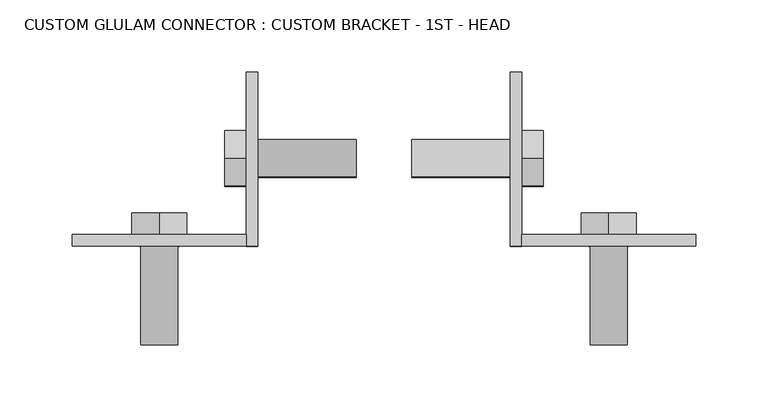
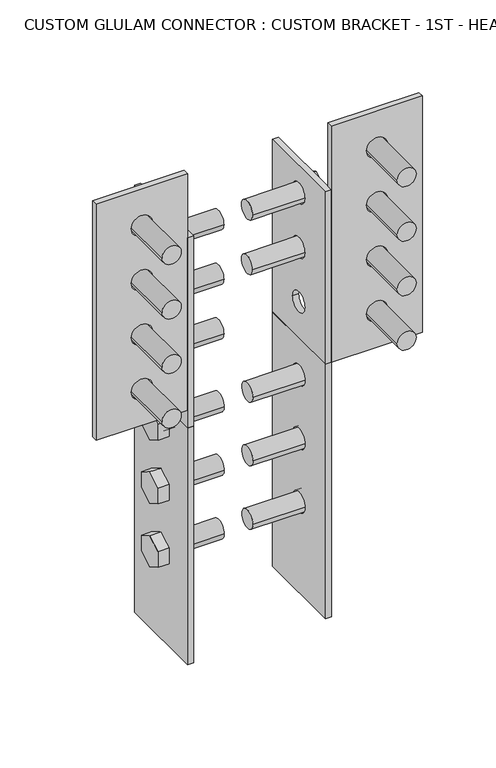
"""IFC4 building model written with IfcOpenShell, lengths in millimetres: fastener geometry, CUSTOM GLULAM CONNECTOR : CUSTOM BRACKET - 1ST - HEAD."""

from ifc_helpers import new_model, si_unit, point, frame, frame_2d, origin, place, context, project, spatial, polyline, circle_curve, trimmed, segment, composite_curve, outline, extrude, source, transform, mapped, element, save
from ifc_brep_helpers import plane_surface, revolved_surface, advanced_brep


def custom_glulam_connector_custom_bracket_1st_head_4a4bef05(model_context):
    return source(origin(), model_context, "Body", "SolidModel", [
        advanced_brep(
        [(-95.25, -60.325, 7.9375), (-87.3125, -60.325, 7.9375), (-87.3125, -60.325, 338.1375), (-95.25, -60.325, 338.1375), (-87.3125, 60.325, 7.9375), (-95.25, 60.325, 7.9375), (-95.25, 60.325, 338.1375), (-87.3125, 60.325, 338.1375), (-95.25, -13.890625, 223.8375), (-95.25, 13.890625, 223.8375), (-87.3125, 13.890625, 223.8375), (-87.3125, -13.890625, 223.8375), (-95.25, 52.3875, 7.9375), (-95.25, 13.890625, 312.7375), (-95.25, -13.890625, 312.7375), (-95.25, -13.890625, 134.9375), (-95.25, 13.890625, 134.9375), (-87.3125, -13.890625, 312.7375), (-87.3125, 13.890625, 312.7375), (-87.3125, 13.890625, 134.9375), (-87.3125, -13.890625, 134.9375)],
        [
            (0, 1),
            (1, 2),
            (2, 3),
            (3, 0),
            (4, 5),
            (5, 6),
            (6, 7),
            (7, 4),
            (8, 9, circle_curve(frame((-95.25, 0.0, 223.8375), z_axis=(-1.0, 0.0, 0.0), x_axis=(0.0, 1.0, 0.0)), 13.890625)),
            (9, 10),
            (10, 11, circle_curve(frame((-87.3125, 0.0, 223.8375), z_axis=(1.0, 0.0, 0.0), x_axis=(0.0, 1.0, 0.0)), 13.890625)),
            (11, 8),
            (5, 12),
            (12, 0),
            (3, 6),
            (8, 9, circle_curve(frame((-95.25, 0.0, 223.8375), z_axis=(1.0, 0.0, 0.0), x_axis=(0.0, 1.0, 0.0)), 13.890625)),
            (13, 14, circle_curve(frame((-95.25, 0.0, 312.7375), z_axis=(1.0, 0.0, 0.0), x_axis=(0.0, 1.0, 0.0)), 13.890625)),
            (14, 13, circle_curve(frame((-95.25, 0.0, 312.7375), z_axis=(1.0, 0.0, 0.0), x_axis=(0.0, 1.0, 0.0)), 13.890625)),
            (15, 16, circle_curve(frame((-95.25, 0.0, 134.9375), z_axis=(1.0, 0.0, 0.0), x_axis=(0.0, 1.0, 0.0)), 13.890625)),
            (16, 15, circle_curve(frame((-95.25, 0.0, 134.9375), z_axis=(1.0, 0.0, 0.0), x_axis=(0.0, 1.0, 0.0)), 13.890625)),
            (14, 17),
            (17, 18, circle_curve(frame((-87.3125, 0.0, 312.7375), z_axis=(1.0, 0.0, 0.0), x_axis=(0.0, 1.0, 0.0)), 13.890625)),
            (18, 13),
            (18, 17, circle_curve(frame((-87.3125, 0.0, 312.7375), z_axis=(1.0, 0.0, 0.0), x_axis=(0.0, 1.0, 0.0)), 13.890625)),
            (11, 10, circle_curve(frame((-87.3125, 0.0, 223.8375), z_axis=(1.0, 0.0, 0.0), x_axis=(0.0, 1.0, 0.0)), 13.890625)),
            (1, 4),
            (7, 2),
            (19, 20, circle_curve(frame((-87.3125, 0.0, 134.9375), z_axis=(-1.0, 0.0, 0.0), x_axis=(0.0, 1.0, 0.0)), 13.890625)),
            (20, 19, circle_curve(frame((-87.3125, 0.0, 134.9375), z_axis=(-1.0, 0.0, 0.0), x_axis=(0.0, 1.0, 0.0)), 13.890625)),
            (15, 20),
            (19, 16),
        ],
        [
            plane_surface(frame((-95.25, -60.325, 363.5375), z_axis=(0.0, -1.0, 0.0), x_axis=(1.0, 0.0, 0.0))),
            plane_surface(frame((-95.25, 60.325, 7.9375), z_axis=(0.0, 1.0, 0.0), x_axis=(1.0, 0.0, 0.0))),
            revolved_surface(polyline([(-95.25, 13.890625, 223.8375), (-87.3125, 13.890625, 223.8375)]), (-87.3125, 0.0, 223.8375), (-1.0, 0.0, 0.0)),
            plane_surface(frame((-95.25, -60.325, 363.5375), z_axis=(-1.0, 0.0, 0.0), x_axis=(0.0, -1.0, 0.0))),
            revolved_surface(polyline([(-95.25, 13.890625, 312.7375), (-87.3125, 13.890625, 312.7375)]), (-87.3125, 0.0, 312.7375), (-1.0, 0.0, 0.0)),
            plane_surface(frame((-87.3125, -60.325, 363.5375), z_axis=(1.0, 0.0, 0.0), x_axis=(0.0, 1.0, 0.0))),
            plane_surface(frame((-95.25, -60.325, 7.9375), z_axis=(0.0, 0.0, -1.0), x_axis=(1.0, 0.0, 0.0))),
            revolved_surface(polyline([(-95.25, 13.890625, 134.9375), (-87.3125, 13.890625, 134.9375)]), (-87.3125, 0.0, 134.9375), (-1.0, 0.0, 0.0)),
            plane_surface(frame((-95.25, -60.325, 338.1375), z_axis=(0.0, 0.0, 1.0), x_axis=(1.0, 0.0, 0.0))),
        ],
        [
            (0, [[1, 2, 3, 4]]),
            (1, [[5, 6, 7, 8]]),
            (2, [[9, 10, 11, 12]]),
            (3, [[13, 14, -4, 15, -6], [-9, 16], [17, 18], [19, 20]]),
            (4, [[-18, 21, 22, 23]]),
            (4, [[-17, -23, 24, -21]]),
            (2, [[-16, -12, 25, -10]]),
            (5, [[26, -8, 27, -2], [-24, -22], [-11, -25], [28, 29]]),
            (6, [[-14, -13, -5, -26, -1]]),
            (7, [[-19, 30, -28, 31]]),
            (7, [[-30, -20, -31, -29]]),
            (8, [[-15, -3, -27, -7]]),
        ],
    ),
        extrude(outline(polyline([(-19.05, 323.7360226), (0.0, 334.7345453), (19.05, 323.7360226), (19.05, 301.7389774), (0.0, 290.7404547), (-19.05, 301.7389774), (-19.05, 323.7360226)])), frame((-110.2320312, 0.0, 0.0), z_axis=(1.0, 0.0, 0.0), x_axis=(0.0, 1.0, 0.0)), (0.0, 0.0, 1.0), 14.9820312),
        extrude(outline(composite_curve([segment(trimmed(circle_curve(frame_2d((0.0, 312.7375)), 12.7), [point((-12.7, 312.7375))], [point((12.7, 312.7375))], False, "CARTESIAN"), True, "CONTINUOUS"), segment(trimmed(circle_curve(frame_2d((0.0, 312.7375)), 12.7), [point((12.7, 312.7375))], [point((-12.7, 312.7375))], False, "CARTESIAN"), True, "CONTINUOUS")], self_intersect=False)), frame((-95.25, 0.0, 0.0), z_axis=(1.0, 0.0, 0.0), x_axis=(0.0, 1.0, 0.0)), (0.0, 0.0, 1.0), 76.2),
        extrude(outline(polyline([(-19.05, 234.8360226), (0.0, 245.8345453), (19.05, 234.8360226), (19.05, 212.8389774), (0.0, 201.8404547), (-19.05, 212.8389774), (-19.05, 234.8360226)])), frame((-110.2320312, 0.0, 0.0), z_axis=(1.0, 0.0, 0.0), x_axis=(0.0, 1.0, 0.0)), (0.0, 0.0, 1.0), 14.9820312),
        extrude(outline(composite_curve([segment(trimmed(circle_curve(frame_2d((0.0, 223.8375)), 12.7), [point((-12.7, 223.8375))], [point((12.7, 223.8375))], False, "CARTESIAN"), True, "CONTINUOUS"), segment(trimmed(circle_curve(frame_2d((0.0, 223.8375)), 12.7), [point((12.7, 223.8375))], [point((-12.7, 223.8375))], False, "CARTESIAN"), True, "CONTINUOUS")], self_intersect=False)), frame((-95.25, 0.0, 0.0), z_axis=(1.0, 0.0, 0.0), x_axis=(0.0, 1.0, 0.0)), (0.0, 0.0, 1.0), 76.2),
        extrude(outline(polyline([(-19.05, 323.7360226), (0.0, 334.7345453), (19.05, 323.7360226), (19.05, 301.7389774), (0.0, 290.7404547), (-19.05, 301.7389774), (-19.05, 323.7360226)])), frame((-110.2320312, 0.0, 0.0), z_axis=(1.0, 0.0, 0.0), x_axis=(0.0, 1.0, 0.0)), (0.0, 0.0, 1.0), 14.9820312),
        extrude(outline(composite_curve([segment(trimmed(circle_curve(frame_2d((0.0, 312.7375)), 12.7), [point((-12.7, 312.7375))], [point((12.7, 312.7375))], False, "CARTESIAN"), True, "CONTINUOUS"), segment(trimmed(circle_curve(frame_2d((0.0, 312.7375)), 12.7), [point((12.7, 312.7375))], [point((-12.7, 312.7375))], False, "CARTESIAN"), True, "CONTINUOUS")], self_intersect=False)), frame((-95.25, 0.0, 0.0), z_axis=(1.0, 0.0, 0.0), x_axis=(0.0, 1.0, 0.0)), (0.0, 0.0, 1.0), 76.2),
        extrude(outline(polyline([(-19.05, 145.9360226), (0.0, 156.9345453), (19.05, 145.9360226), (19.05, 123.9389774), (0.0, 112.9404547), (-19.05, 123.9389774), (-19.05, 145.9360226)])), frame((-110.2320312, 0.0, 0.0), z_axis=(1.0, 0.0, 0.0), x_axis=(0.0, 1.0, 0.0)), (0.0, 0.0, 1.0), 14.9820312),
        extrude(outline(composite_curve([segment(trimmed(circle_curve(frame_2d((0.0, 134.9375)), 12.7), [point((-12.7, 134.9375))], [point((12.7, 134.9375))], False, "CARTESIAN"), True, "CONTINUOUS"), segment(trimmed(circle_curve(frame_2d((0.0, 134.9375)), 12.7), [point((12.7, 134.9375))], [point((-12.7, 134.9375))], False, "CARTESIAN"), True, "CONTINUOUS")], self_intersect=False)), frame((-95.25, 0.0, 0.0), z_axis=(1.0, 0.0, 0.0), x_axis=(0.0, 1.0, 0.0)), (0.0, 0.0, 1.0), 76.2),
        advanced_brep(
        [(95.25, -60.325, 7.9375), (95.25, -60.325, 363.5375), (87.3125, -60.325, 363.5375), (87.3125, -60.325, 7.9375), (95.25, 60.325, 363.5375), (95.25, 60.325, 7.9375), (87.3125, 60.325, 7.9375), (87.3125, 60.325, 363.5375), (95.25, -13.890625, 223.8375), (87.3125, -13.890625, 223.8375), (87.3125, 13.890625, 223.8375), (95.25, 13.890625, 223.8375), (95.25, 52.3875, 363.5375), (95.25, 52.3875, 7.9375), (95.25, 13.890625, 312.7375), (95.25, -13.890625, 312.7375), (95.25, 13.890625, 134.9375), (95.25, -13.890625, 134.9375), (87.3125, -13.890625, 312.7375), (87.3125, 13.890625, 312.7375), (87.3125, -13.890625, 134.9375), (87.3125, 13.890625, 134.9375)],
        [
            (0, 1),
            (1, 2),
            (2, 3),
            (3, 0),
            (4, 5),
            (5, 6),
            (6, 7),
            (7, 4),
            (8, 9),
            (9, 10, circle_curve(frame((87.3125, 0.0, 223.8375), z_axis=(-1.0, 0.0, 0.0), x_axis=(0.0, 1.0, 0.0)), 13.890625)),
            (10, 11),
            (11, 8, circle_curve(frame((95.25, 0.0, 223.8375), z_axis=(1.0, 0.0, 0.0), x_axis=(0.0, 1.0, 0.0)), 13.890625)),
            (4, 12),
            (12, 1),
            (0, 13),
            (13, 5),
            (14, 15, circle_curve(frame((95.25, 0.0, 312.7375), z_axis=(-1.0, 0.0, 0.0), x_axis=(0.0, 1.0, 0.0)), 13.890625)),
            (15, 14, circle_curve(frame((95.25, 0.0, 312.7375), z_axis=(-1.0, 0.0, 0.0), x_axis=(0.0, 1.0, 0.0)), 13.890625)),
            (11, 8, circle_curve(frame((95.25, 0.0, 223.8375), z_axis=(-1.0, 0.0, 0.0), x_axis=(0.0, 1.0, 0.0)), 13.890625)),
            (16, 17, circle_curve(frame((95.25, 0.0, 134.9375), z_axis=(-1.0, 0.0, 0.0), x_axis=(0.0, 1.0, 0.0)), 13.890625)),
            (17, 16, circle_curve(frame((95.25, 0.0, 134.9375), z_axis=(-1.0, 0.0, 0.0), x_axis=(0.0, 1.0, 0.0)), 13.890625)),
            (18, 15),
            (14, 19),
            (19, 18, circle_curve(frame((87.3125, 0.0, 312.7375), z_axis=(-1.0, 0.0, 0.0), x_axis=(0.0, 1.0, 0.0)), 13.890625)),
            (18, 19, circle_curve(frame((87.3125, 0.0, 312.7375), z_axis=(-1.0, 0.0, 0.0), x_axis=(0.0, 1.0, 0.0)), 13.890625)),
            (10, 9, circle_curve(frame((87.3125, 0.0, 223.8375), z_axis=(-1.0, 0.0, 0.0), x_axis=(0.0, 1.0, 0.0)), 13.890625)),
            (6, 3),
            (2, 7),
            (20, 21, circle_curve(frame((87.3125, 0.0, 134.9375), z_axis=(1.0, 0.0, 0.0), x_axis=(0.0, 1.0, 0.0)), 13.890625)),
            (21, 20, circle_curve(frame((87.3125, 0.0, 134.9375), z_axis=(1.0, 0.0, 0.0), x_axis=(0.0, 1.0, 0.0)), 13.890625)),
            (20, 17),
            (16, 21),
        ],
        [
            plane_surface(frame((95.25, -60.325, 363.5375), z_axis=(0.0, -1.0, 0.0), x_axis=(-1.0, 0.0, 0.0))),
            plane_surface(frame((95.25, 60.325, 7.9375), z_axis=(0.0, 1.0, 0.0), x_axis=(-1.0, 0.0, 0.0))),
            revolved_surface(polyline([(95.25, 13.890625, 223.8375), (87.3125, 13.890625, 223.8375)]), (87.3125, 0.0, 223.8375), (1.0, 0.0, 0.0)),
            plane_surface(frame((95.25, -60.325, 363.5375), z_axis=(1.0, 0.0, 0.0), x_axis=(0.0, -1.0, 0.0))),
            revolved_surface(polyline([(95.25, 13.890625, 312.7375), (87.3125, 13.890625, 312.7375)]), (87.3125, 0.0, 312.7375), (1.0, 0.0, 0.0)),
            plane_surface(frame((87.3125, -60.325, 363.5375), z_axis=(-1.0, 0.0, 0.0), x_axis=(0.0, 1.0, 0.0))),
            plane_surface(frame((95.25, 60.325, 363.5375), z_axis=(0.0, 0.0, 1.0), x_axis=(-1.0, 0.0, 0.0))),
            plane_surface(frame((95.25, -60.325, 7.9375), z_axis=(0.0, 0.0, -1.0), x_axis=(-1.0, 0.0, 0.0))),
            revolved_surface(polyline([(95.25, 13.890625, 134.9375), (87.3125, 13.890625, 134.9375)]), (87.3125, 0.0, 134.9375), (1.0, 0.0, 0.0)),
        ],
        [
            (0, [[1, 2, 3, 4]]),
            (1, [[5, 6, 7, 8]]),
            (2, [[9, 10, 11, 12]]),
            (3, [[13, 14, -1, 15, 16, -5], [17, 18], [19, -12], [20, 21]]),
            (4, [[22, -17, 23, 24]]),
            (4, [[-22, 25, -23, -18]]),
            (2, [[-9, -19, -11, 26]]),
            (5, [[-7, 27, -3, 28], [-24, -25], [-26, -10], [29, 30]]),
            (6, [[-14, -13, -8, -28, -2]]),
            (7, [[-16, -15, -4, -27, -6]]),
            (8, [[31, -20, 32, -29]]),
            (8, [[-31, -30, -32, -21]]),
        ],
    ),
        extrude(outline(polyline([(-19.05, 323.7360226), (0.0, 334.7345453), (19.05, 323.7360226), (19.05, 301.7389774), (0.0, 290.7404547), (-19.05, 301.7389774), (-19.05, 323.7360226)])), frame((95.25, 0.0, 0.0), z_axis=(1.0, 0.0, 0.0), x_axis=(0.0, 1.0, 0.0)), (0.0, 0.0, 1.0), 14.9820312),
        extrude(outline(composite_curve([segment(trimmed(circle_curve(frame_2d((0.0, 312.7375)), 12.7), [point((-12.7, 312.7375))], [point((12.7, 312.7375))], False, "CARTESIAN"), True, "CONTINUOUS"), segment(trimmed(circle_curve(frame_2d((0.0, 312.7375)), 12.7), [point((12.7, 312.7375))], [point((-12.7, 312.7375))], False, "CARTESIAN"), True, "CONTINUOUS")], self_intersect=False)), frame((19.05, 0.0, 0.0), z_axis=(1.0, 0.0, 0.0), x_axis=(0.0, 1.0, 0.0)), (0.0, 0.0, 1.0), 76.2),
        extrude(outline(polyline([(-19.05, 234.8360226), (0.0, 245.8345453), (19.05, 234.8360226), (19.05, 212.8389774), (0.0, 201.8404547), (-19.05, 212.8389774), (-19.05, 234.8360226)])), frame((95.25, 0.0, 0.0), z_axis=(1.0, 0.0, 0.0), x_axis=(0.0, 1.0, 0.0)), (0.0, 0.0, 1.0), 14.9820312),
        extrude(outline(composite_curve([segment(trimmed(circle_curve(frame_2d((0.0, 223.8375)), 12.7), [point((-12.7, 223.8375))], [point((12.7, 223.8375))], False, "CARTESIAN"), True, "CONTINUOUS"), segment(trimmed(circle_curve(frame_2d((0.0, 223.8375)), 12.7), [point((12.7, 223.8375))], [point((-12.7, 223.8375))], False, "CARTESIAN"), True, "CONTINUOUS")], self_intersect=False)), frame((19.05, 0.0, 0.0), z_axis=(1.0, 0.0, 0.0), x_axis=(0.0, 1.0, 0.0)), (0.0, 0.0, 1.0), 76.2),
        extrude(outline(polyline([(-19.05, 323.7360226), (0.0, 334.7345453), (19.05, 323.7360226), (19.05, 301.7389774), (0.0, 290.7404547), (-19.05, 301.7389774), (-19.05, 323.7360226)])), frame((95.25, 0.0, 0.0), z_axis=(1.0, 0.0, 0.0), x_axis=(0.0, 1.0, 0.0)), (0.0, 0.0, 1.0), 14.9820312),
        extrude(outline(composite_curve([segment(trimmed(circle_curve(frame_2d((0.0, 312.7375)), 12.7), [point((-12.7, 312.7375))], [point((12.7, 312.7375))], False, "CARTESIAN"), True, "CONTINUOUS"), segment(trimmed(circle_curve(frame_2d((0.0, 312.7375)), 12.7), [point((12.7, 312.7375))], [point((-12.7, 312.7375))], False, "CARTESIAN"), True, "CONTINUOUS")], self_intersect=False)), frame((19.05, 0.0, 0.0), z_axis=(1.0, 0.0, 0.0), x_axis=(0.0, 1.0, 0.0)), (0.0, 0.0, 1.0), 76.2),
        extrude(outline(polyline([(-19.05, 145.9360226), (0.0, 156.9345453), (19.05, 145.9360226), (19.05, 123.9389774), (0.0, 112.9404547), (-19.05, 123.9389774), (-19.05, 145.9360226)])), frame((95.25, 0.0, 0.0), z_axis=(1.0, 0.0, 0.0), x_axis=(0.0, 1.0, 0.0)), (0.0, 0.0, 1.0), 14.9820312),
        extrude(outline(composite_curve([segment(trimmed(circle_curve(frame_2d((0.0, 134.9375)), 12.7), [point((-12.7, 134.9375))], [point((12.7, 134.9375))], False, "CARTESIAN"), True, "CONTINUOUS"), segment(trimmed(circle_curve(frame_2d((0.0, 134.9375)), 12.7), [point((12.7, 134.9375))], [point((-12.7, 134.9375))], False, "CARTESIAN"), True, "CONTINUOUS")], self_intersect=False)), frame((19.05, 0.0, 0.0), z_axis=(1.0, 0.0, 0.0), x_axis=(0.0, 1.0, 0.0)), (0.0, 0.0, 1.0), 76.2),
        advanced_brep(
        [(-215.9, -52.3875, 693.7375), (-215.9, -52.3875, 363.5375), (-215.9, -60.325, 363.5375), (-215.9, -60.325, 693.7375), (-141.684375, -60.325, 642.9375), (-141.684375, -52.3875, 642.9375), (-169.465625, -52.3875, 642.9375), (-169.465625, -60.325, 642.9375), (-95.25, -52.3875, 693.7375), (-95.25, -52.3875, 363.5375), (-169.465625, -52.3875, 566.7375), (-141.684375, -52.3875, 566.7375), (-169.465625, -52.3875, 490.5375), (-141.684375, -52.3875, 490.5375), (-169.465625, -52.3875, 414.3375), (-141.684375, -52.3875, 414.3375), (-95.25, -60.325, 693.7375), (-95.25, -60.325, 604.8375), (-95.25, -60.325, 363.5375), (-141.684375, -60.325, 566.7375), (-169.465625, -60.325, 566.7375), (-141.684375, -60.325, 490.5375), (-169.465625, -60.325, 490.5375), (-141.684375, -60.325, 414.3375), (-169.465625, -60.325, 414.3375)],
        [
            (0, 1),
            (1, 2),
            (2, 3),
            (3, 0),
            (4, 5),
            (5, 6, circle_curve(frame((-155.575, -52.3875, 642.9375), z_axis=(0.0, 1.0, 0.0), x_axis=(-1.0, 0.0, 0.0)), 13.890625)),
            (6, 7),
            (7, 4, circle_curve(frame((-155.575, -60.325, 642.9375), z_axis=(0.0, -1.0, 0.0), x_axis=(-1.0, 0.0, 0.0)), 13.890625)),
            (4, 7, circle_curve(frame((-155.575, -60.325, 642.9375), z_axis=(0.0, -1.0, 0.0), x_axis=(-1.0, 0.0, 0.0)), 13.890625)),
            (6, 5, circle_curve(frame((-155.575, -52.3875, 642.9375), z_axis=(0.0, 1.0, 0.0), x_axis=(-1.0, 0.0, 0.0)), 13.890625)),
            (0, 8),
            (8, 9),
            (9, 1),
            (10, 11, circle_curve(frame((-155.575, -52.3875, 566.7375), z_axis=(0.0, -1.0, 0.0), x_axis=(-1.0, 0.0, 0.0)), 13.890625)),
            (11, 10, circle_curve(frame((-155.575, -52.3875, 566.7375), z_axis=(0.0, -1.0, 0.0), x_axis=(-1.0, 0.0, 0.0)), 13.890625)),
            (12, 13, circle_curve(frame((-155.575, -52.3875, 490.5375), z_axis=(0.0, -1.0, 0.0), x_axis=(-1.0, 0.0, 0.0)), 13.890625)),
            (13, 12, circle_curve(frame((-155.575, -52.3875, 490.5375), z_axis=(0.0, -1.0, 0.0), x_axis=(-1.0, 0.0, 0.0)), 13.890625)),
            (14, 15, circle_curve(frame((-155.575, -52.3875, 414.3375), z_axis=(0.0, -1.0, 0.0), x_axis=(-1.0, 0.0, 0.0)), 13.890625)),
            (15, 14, circle_curve(frame((-155.575, -52.3875, 414.3375), z_axis=(0.0, -1.0, 0.0), x_axis=(-1.0, 0.0, 0.0)), 13.890625)),
            (8, 16),
            (16, 17),
            (17, 18),
            (18, 9),
            (18, 2),
            (16, 3),
            (19, 20, circle_curve(frame((-155.575, -60.325, 566.7375), z_axis=(0.0, 1.0, 0.0), x_axis=(-1.0, 0.0, 0.0)), 13.890625)),
            (20, 19, circle_curve(frame((-155.575, -60.325, 566.7375), z_axis=(0.0, 1.0, 0.0), x_axis=(-1.0, 0.0, 0.0)), 13.890625)),
            (21, 22, circle_curve(frame((-155.575, -60.325, 490.5375), z_axis=(0.0, 1.0, 0.0), x_axis=(-1.0, 0.0, 0.0)), 13.890625)),
            (22, 21, circle_curve(frame((-155.575, -60.325, 490.5375), z_axis=(0.0, 1.0, 0.0), x_axis=(-1.0, 0.0, 0.0)), 13.890625)),
            (23, 24, circle_curve(frame((-155.575, -60.325, 414.3375), z_axis=(0.0, 1.0, 0.0), x_axis=(-1.0, 0.0, 0.0)), 13.890625)),
            (24, 23, circle_curve(frame((-155.575, -60.325, 414.3375), z_axis=(0.0, 1.0, 0.0), x_axis=(-1.0, 0.0, 0.0)), 13.890625)),
            (19, 11),
            (10, 20),
            (13, 21),
            (22, 12),
            (23, 15),
            (14, 24),
        ],
        [
            plane_surface(frame((-215.9, -52.3875, 363.5375), z_axis=(-1.0, 0.0, 0.0), x_axis=(0.0, -1.0, 0.0))),
            revolved_surface(polyline([(-169.465625, -52.3875, 642.9375), (-169.465625, -60.325, 642.9375)]), (-155.575, -60.325, 642.9375), (0.0, 1.0, 0.0)),
            plane_surface(frame((-95.25, -52.3875, 693.7375), z_axis=(0.0, 1.0, 0.0), x_axis=(1.0, 0.0, 0.0))),
            plane_surface(frame((-95.25, -52.3875, 693.7375), z_axis=(1.0, 0.0, 0.0), x_axis=(0.0, -1.0, 0.0))),
            plane_surface(frame((-95.25, -52.3875, 363.5375), z_axis=(0.0, 0.0, -1.0), x_axis=(0.0, -1.0, 0.0))),
            plane_surface(frame((-95.25, -60.325, 693.7375), z_axis=(0.0, -1.0, 0.0), x_axis=(-1.0, 0.0, 0.0))),
            plane_surface(frame((-215.9, -52.3875, 693.7375), z_axis=(0.0, 0.0, 1.0), x_axis=(0.0, -1.0, 0.0))),
            revolved_surface(polyline([(-169.465625, -52.3875, 566.7375), (-169.465625, -60.325, 566.7375)]), (-155.575, -60.325, 566.7375), (0.0, 1.0, 0.0)),
            revolved_surface(polyline([(-169.465625, -52.3875, 490.5375), (-169.465625, -60.325, 490.5375)]), (-155.575, -60.325, 490.5375), (0.0, 1.0, 0.0)),
            revolved_surface(polyline([(-169.465625, -52.3875, 414.3375), (-169.465625, -60.325, 414.3375)]), (-155.575, -60.325, 414.3375), (0.0, 1.0, 0.0)),
        ],
        [
            (0, [[1, 2, 3, 4]]),
            (1, [[5, 6, 7, 8]]),
            (1, [[-5, 9, -7, 10]]),
            (2, [[11, 12, 13, -1], [14, 15], [-6, -10], [16, 17], [18, 19]]),
            (3, [[-12, 20, 21, 22, 23]]),
            (4, [[-13, -23, 24, -2]]),
            (5, [[-3, -24, -22, -21, 25], [-8, -9], [26, 27], [28, 29], [30, 31]]),
            (6, [[-11, -4, -25, -20]]),
            (7, [[32, -14, 33, -26]]),
            (7, [[-32, -27, -33, -15]]),
            (8, [[34, -29, 35, -17]]),
            (8, [[-34, -16, -35, -28]]),
            (9, [[36, -18, 37, -30]]),
            (9, [[-36, -31, -37, -19]]),
        ],
    ),
        extrude(outline(polyline([(653.9360226, -136.525), (664.9345453, -155.575), (653.9360226, -174.625), (631.9389774, -174.625), (620.9404547, -155.575), (631.9389774, -136.525), (653.9360226, -136.525)])), frame((0.0, -52.3875, 0.0), z_axis=(0.0, 1.0, 0.0), x_axis=(0.0, 0.0, 1.0)), (0.0, 0.0, 1.0), 14.9820312),
        extrude(outline(composite_curve([segment(trimmed(circle_curve(frame_2d((642.9375, -155.575)), 12.7), [point((642.9375, -142.875))], [point((642.9375, -168.275))], False, "CARTESIAN"), True, "CONTINUOUS"), segment(trimmed(circle_curve(frame_2d((642.9375, -155.575)), 12.7), [point((642.9375, -168.275))], [point((642.9375, -142.875))], False, "CARTESIAN"), True, "CONTINUOUS")], self_intersect=False)), frame((0.0, -128.5875, 0.0), z_axis=(0.0, 1.0, 0.0), x_axis=(0.0, 0.0, 1.0)), (0.0, 0.0, 1.0), 76.2),
        extrude(outline(polyline([(577.7360226, -136.525), (588.7345453, -155.575), (577.7360226, -174.625), (555.7389774, -174.625), (544.7404547, -155.575), (555.7389774, -136.525), (577.7360226, -136.525)])), frame((0.0, -52.3875, 0.0), z_axis=(0.0, 1.0, 0.0), x_axis=(0.0, 0.0, 1.0)), (0.0, 0.0, 1.0), 14.9820312),
        extrude(outline(composite_curve([segment(trimmed(circle_curve(frame_2d((566.7375, -155.575)), 12.7), [point((566.7375, -142.875))], [point((566.7375, -168.275))], False, "CARTESIAN"), True, "CONTINUOUS"), segment(trimmed(circle_curve(frame_2d((566.7375, -155.575)), 12.7), [point((566.7375, -168.275))], [point((566.7375, -142.875))], False, "CARTESIAN"), True, "CONTINUOUS")], self_intersect=False)), frame((0.0, -128.5875, 0.0), z_axis=(0.0, 1.0, 0.0), x_axis=(0.0, 0.0, 1.0)), (0.0, 0.0, 1.0), 76.2),
        extrude(outline(polyline([(653.9360226, -136.525), (664.9345453, -155.575), (653.9360226, -174.625), (631.9389774, -174.625), (620.9404547, -155.575), (631.9389774, -136.525), (653.9360226, -136.525)])), frame((0.0, -52.3875, 0.0), z_axis=(0.0, 1.0, 0.0), x_axis=(0.0, 0.0, 1.0)), (0.0, 0.0, 1.0), 14.9820312),
        extrude(outline(composite_curve([segment(trimmed(circle_curve(frame_2d((642.9375, -155.575)), 12.7), [point((642.9375, -142.875))], [point((642.9375, -168.275))], False, "CARTESIAN"), True, "CONTINUOUS"), segment(trimmed(circle_curve(frame_2d((642.9375, -155.575)), 12.7), [point((642.9375, -168.275))], [point((642.9375, -142.875))], False, "CARTESIAN"), True, "CONTINUOUS")], self_intersect=False)), frame((0.0, -128.5875, 0.0), z_axis=(0.0, 1.0, 0.0), x_axis=(0.0, 0.0, 1.0)), (0.0, 0.0, 1.0), 76.2),
        extrude(outline(polyline([(501.5360226, -136.525), (512.5345453, -155.575), (501.5360226, -174.625), (479.5389774, -174.625), (468.5404547, -155.575), (479.5389774, -136.525), (501.5360226, -136.525)])), frame((0.0, -52.3875, 0.0), z_axis=(0.0, 1.0, 0.0), x_axis=(0.0, 0.0, 1.0)), (0.0, 0.0, 1.0), 14.9820312),
        extrude(outline(composite_curve([segment(trimmed(circle_curve(frame_2d((490.5375, -155.575)), 12.7), [point((490.5375, -142.875))], [point((490.5375, -168.275))], False, "CARTESIAN"), True, "CONTINUOUS"), segment(trimmed(circle_curve(frame_2d((490.5375, -155.575)), 12.7), [point((490.5375, -168.275))], [point((490.5375, -142.875))], False, "CARTESIAN"), True, "CONTINUOUS")], self_intersect=False)), frame((0.0, -128.5875, 0.0), z_axis=(0.0, 1.0, 0.0), x_axis=(0.0, 0.0, 1.0)), (0.0, 0.0, 1.0), 76.2),
        extrude(outline(polyline([(425.3360226, -136.525), (436.3345453, -155.575), (425.3360226, -174.625), (403.3389774, -174.625), (392.3404547, -155.575), (403.3389774, -136.525), (425.3360226, -136.525)])), frame((0.0, -52.3875, 0.0), z_axis=(0.0, 1.0, 0.0), x_axis=(0.0, 0.0, 1.0)), (0.0, 0.0, 1.0), 14.9820312),
        extrude(outline(composite_curve([segment(trimmed(circle_curve(frame_2d((414.3375, -155.575)), 12.7), [point((414.3375, -142.875))], [point((414.3375, -168.275))], False, "CARTESIAN"), True, "CONTINUOUS"), segment(trimmed(circle_curve(frame_2d((414.3375, -155.575)), 12.7), [point((414.3375, -168.275))], [point((414.3375, -142.875))], False, "CARTESIAN"), True, "CONTINUOUS")], self_intersect=False)), frame((0.0, -128.5875, 0.0), z_axis=(0.0, 1.0, 0.0), x_axis=(0.0, 0.0, 1.0)), (0.0, 0.0, 1.0), 76.2),
        advanced_brep(
        [(-95.25, -60.325, 338.1375), (-87.3125, -60.325, 338.1375), (-87.3125, -60.325, 604.8375), (-95.25, -60.325, 604.8375), (-95.25, -60.325, 363.5375), (-95.25, 60.325, 604.8375), (-87.3125, 60.325, 604.8375), (-87.3125, 60.325, 338.1375), (-95.25, 60.325, 338.1375), (-95.25, -13.096875, 490.5375), (-95.25, 14.684375, 490.5375), (-87.3125, 14.684375, 490.5375), (-87.3125, -13.096875, 490.5375), (-95.25, 14.684375, 566.7375), (-95.25, -13.096875, 566.7375), (-95.25, 14.684375, 414.3375), (-95.25, -13.096875, 414.3375), (-87.3125, -13.096875, 566.7375), (-87.3125, 14.684375, 566.7375), (-87.3125, -13.096875, 414.3375), (-87.3125, 14.684375, 414.3375)],
        [
            (0, 1),
            (1, 2),
            (2, 3),
            (3, 4),
            (4, 0),
            (5, 6),
            (6, 7),
            (7, 8),
            (8, 5),
            (9, 10, circle_curve(frame((-95.25, 0.79375, 490.5375), z_axis=(-1.0, 0.0, 0.0), x_axis=(0.0, 1.0, 0.0)), 13.890625)),
            (10, 11),
            (11, 12, circle_curve(frame((-87.3125, 0.79375, 490.5375), z_axis=(1.0, 0.0, 0.0), x_axis=(0.0, 1.0, 0.0)), 13.890625)),
            (12, 9),
            (8, 0),
            (3, 5),
            (9, 10, circle_curve(frame((-95.25, 0.79375, 490.5375), z_axis=(1.0, 0.0, 0.0), x_axis=(0.0, 1.0, 0.0)), 13.890625)),
            (13, 14, circle_curve(frame((-95.25, 0.79375, 566.7375), z_axis=(1.0, 0.0, 0.0), x_axis=(0.0, 1.0, 0.0)), 13.890625)),
            (14, 13, circle_curve(frame((-95.25, 0.79375, 566.7375), z_axis=(1.0, 0.0, 0.0), x_axis=(0.0, 1.0, 0.0)), 13.890625)),
            (15, 16, circle_curve(frame((-95.25, 0.79375, 414.3375), z_axis=(1.0, 0.0, 0.0), x_axis=(0.0, 1.0, 0.0)), 13.890625)),
            (16, 15, circle_curve(frame((-95.25, 0.79375, 414.3375), z_axis=(1.0, 0.0, 0.0), x_axis=(0.0, 1.0, 0.0)), 13.890625)),
            (17, 18, circle_curve(frame((-87.3125, 0.79375, 566.7375), z_axis=(1.0, 0.0, 0.0), x_axis=(0.0, 1.0, 0.0)), 13.890625)),
            (18, 13),
            (14, 17),
            (18, 17, circle_curve(frame((-87.3125, 0.79375, 566.7375), z_axis=(1.0, 0.0, 0.0), x_axis=(0.0, 1.0, 0.0)), 13.890625)),
            (12, 11, circle_curve(frame((-87.3125, 0.79375, 490.5375), z_axis=(1.0, 0.0, 0.0), x_axis=(0.0, 1.0, 0.0)), 13.890625)),
            (6, 2),
            (1, 7),
            (19, 20, circle_curve(frame((-87.3125, 0.79375, 414.3375), z_axis=(-1.0, 0.0, 0.0), x_axis=(0.0, 1.0, 0.0)), 13.890625)),
            (20, 19, circle_curve(frame((-87.3125, 0.79375, 414.3375), z_axis=(-1.0, 0.0, 0.0), x_axis=(0.0, 1.0, 0.0)), 13.890625)),
            (20, 15),
            (16, 19),
        ],
        [
            plane_surface(frame((-95.25, -60.325, 604.8375), z_axis=(0.0, -1.0, 0.0), x_axis=(1.0, 0.0, 0.0))),
            plane_surface(frame((-95.25, 60.325, 338.1375), z_axis=(0.0, 1.0, 0.0), x_axis=(1.0, 0.0, 0.0))),
            revolved_surface(polyline([(-95.25, 14.684375, 490.5375), (-87.3125, 14.684375, 490.5375)]), (-87.3125, 0.79375, 490.5375), (-1.0, 0.0, 0.0)),
            plane_surface(frame((-95.25, -60.325, 604.8375), z_axis=(-1.0, 0.0, 0.0), x_axis=(0.0, -1.0, 0.0))),
            revolved_surface(polyline([(-95.25, 14.684375, 566.7375), (-87.3125, 14.684375, 566.7375)]), (-87.3125, 0.79375, 566.7375), (-1.0, 0.0, 0.0)),
            plane_surface(frame((-87.3125, -60.325, 604.8375), z_axis=(1.0, 0.0, 0.0), x_axis=(0.0, 1.0, 0.0))),
            plane_surface(frame((-95.25, 60.325, 604.8375), z_axis=(0.0, 0.0, 1.0), x_axis=(1.0, 0.0, 0.0))),
            plane_surface(frame((-95.25, -60.325, 338.1375), z_axis=(0.0, 0.0, -1.0), x_axis=(1.0, 0.0, 0.0))),
            revolved_surface(polyline([(-95.25, 14.684375, 414.3375), (-87.3125, 14.684375, 414.3375)]), (-87.3125, 0.79375, 414.3375), (-1.0, 0.0, 0.0)),
        ],
        [
            (0, [[1, 2, 3, 4, 5]]),
            (1, [[6, 7, 8, 9]]),
            (2, [[10, 11, 12, 13]]),
            (3, [[-9, 14, -5, -4, 15], [-10, 16], [17, 18], [19, 20]]),
            (4, [[21, 22, -18, 23]]),
            (4, [[-17, -22, 24, -23]]),
            (2, [[25, -11, -16, -13]]),
            (5, [[26, -2, 27, -7], [-24, -21], [-12, -25], [28, 29]]),
            (6, [[-3, -26, -6, -15]]),
            (7, [[-8, -27, -1, -14]]),
            (8, [[-29, 30, -20, 31]]),
            (8, [[-19, -30, -28, -31]]),
        ],
    ),
        extrude(outline(polyline([(-18.25625, 577.7360226), (0.79375, 588.7345453), (19.84375, 577.7360226), (19.84375, 555.7389774), (0.79375, 544.7404547), (-18.25625, 555.7389774), (-18.25625, 577.7360226)])), frame((-110.2320312, 0.0, 0.0), z_axis=(1.0, 0.0, 0.0), x_axis=(0.0, 1.0, 0.0)), (0.0, 0.0, 1.0), 14.9820312),
        extrude(outline(composite_curve([segment(trimmed(circle_curve(frame_2d((0.79375, 566.7375)), 12.7), [point((-11.90625, 566.7375))], [point((13.49375, 566.7375))], False, "CARTESIAN"), True, "CONTINUOUS"), segment(trimmed(circle_curve(frame_2d((0.79375, 566.7375)), 12.7), [point((13.49375, 566.7375))], [point((-11.90625, 566.7375))], False, "CARTESIAN"), True, "CONTINUOUS")], self_intersect=False)), frame((-95.25, 0.0, 0.0), z_axis=(1.0, 0.0, 0.0), x_axis=(0.0, 1.0, 0.0)), (0.0, 0.0, 1.0), 76.2),
        extrude(outline(polyline([(-18.25625, 501.5360226), (0.79375, 512.5345453), (19.84375, 501.5360226), (19.84375, 479.5389774), (0.79375, 468.5404547), (-18.25625, 479.5389774), (-18.25625, 501.5360226)])), frame((-110.2320312, 0.0, 0.0), z_axis=(1.0, 0.0, 0.0), x_axis=(0.0, 1.0, 0.0)), (0.0, 0.0, 1.0), 14.9820312),
        extrude(outline(composite_curve([segment(trimmed(circle_curve(frame_2d((0.79375, 490.5375)), 12.7), [point((-11.90625, 490.5375))], [point((13.49375, 490.5375))], False, "CARTESIAN"), True, "CONTINUOUS"), segment(trimmed(circle_curve(frame_2d((0.79375, 490.5375)), 12.7), [point((13.49375, 490.5375))], [point((-11.90625, 490.5375))], False, "CARTESIAN"), True, "CONTINUOUS")], self_intersect=False)), frame((-95.25, 0.0, 0.0), z_axis=(1.0, 0.0, 0.0), x_axis=(0.0, 1.0, 0.0)), (0.0, 0.0, 1.0), 76.2),
        extrude(outline(polyline([(-18.25625, 577.7360226), (0.79375, 588.7345453), (19.84375, 577.7360226), (19.84375, 555.7389774), (0.79375, 544.7404547), (-18.25625, 555.7389774), (-18.25625, 577.7360226)])), frame((-110.2320312, 0.0, 0.0), z_axis=(1.0, 0.0, 0.0), x_axis=(0.0, 1.0, 0.0)), (0.0, 0.0, 1.0), 14.9820312),
        extrude(outline(composite_curve([segment(trimmed(circle_curve(frame_2d((0.79375, 566.7375)), 12.7), [point((-11.90625, 566.7375))], [point((13.49375, 566.7375))], False, "CARTESIAN"), True, "CONTINUOUS"), segment(trimmed(circle_curve(frame_2d((0.79375, 566.7375)), 12.7), [point((13.49375, 566.7375))], [point((-11.90625, 566.7375))], False, "CARTESIAN"), True, "CONTINUOUS")], self_intersect=False)), frame((-95.25, 0.0, 0.0), z_axis=(1.0, 0.0, 0.0), x_axis=(0.0, 1.0, 0.0)), (0.0, 0.0, 1.0), 76.2),
        extrude(outline(polyline([(-18.25625, 425.3360226), (0.79375, 436.3345453), (19.84375, 425.3360226), (19.84375, 403.3389774), (0.79375, 392.3404547), (-18.25625, 403.3389774), (-18.25625, 425.3360226)])), frame((-110.2320312, 0.0, 0.0), z_axis=(1.0, 0.0, 0.0), x_axis=(0.0, 1.0, 0.0)), (0.0, 0.0, 1.0), 14.9820312),
        extrude(outline(composite_curve([segment(trimmed(circle_curve(frame_2d((0.79375, 414.3375)), 12.7), [point((-11.90625, 414.3375))], [point((13.49375, 414.3375))], False, "CARTESIAN"), True, "CONTINUOUS"), segment(trimmed(circle_curve(frame_2d((0.79375, 414.3375)), 12.7), [point((13.49375, 414.3375))], [point((-11.90625, 414.3375))], False, "CARTESIAN"), True, "CONTINUOUS")], self_intersect=False)), frame((-95.25, 0.0, 0.0), z_axis=(1.0, 0.0, 0.0), x_axis=(0.0, 1.0, 0.0)), (0.0, 0.0, 1.0), 76.2),
        advanced_brep(
        [(215.9, -52.3875, 693.7375), (215.9, -60.325, 693.7375), (215.9, -60.325, 363.5375), (215.9, -52.3875, 363.5375), (141.684375, -60.325, 642.9375), (169.465625, -60.325, 642.9375), (169.465625, -52.3875, 642.9375), (141.684375, -52.3875, 642.9375), (95.25, -52.3875, 363.5375), (95.25, -52.3875, 693.7375), (169.465625, -52.3875, 566.7375), (141.684375, -52.3875, 566.7375), (169.465625, -52.3875, 490.5375), (141.684375, -52.3875, 490.5375), (169.465625, -52.3875, 414.3375), (141.684375, -52.3875, 414.3375), (95.25, -60.325, 363.5375), (95.25, -60.325, 604.8375), (95.25, -60.325, 693.7375), (141.684375, -60.325, 566.7375), (169.465625, -60.325, 566.7375), (141.684375, -60.325, 490.5375), (169.465625, -60.325, 490.5375), (141.684375, -60.325, 414.3375), (169.465625, -60.325, 414.3375)],
        [
            (0, 1),
            (1, 2),
            (2, 3),
            (3, 0),
            (4, 5, circle_curve(frame((155.575, -60.325, 642.9375), z_axis=(0.0, -1.0, 0.0), x_axis=(1.0, 0.0, 0.0)), 13.890625)),
            (5, 6),
            (6, 7, circle_curve(frame((155.575, -52.3875, 642.9375), z_axis=(0.0, 1.0, 0.0), x_axis=(1.0, 0.0, 0.0)), 13.890625)),
            (7, 4),
            (7, 6, circle_curve(frame((155.575, -52.3875, 642.9375), z_axis=(0.0, 1.0, 0.0), x_axis=(1.0, 0.0, 0.0)), 13.890625)),
            (5, 4, circle_curve(frame((155.575, -60.325, 642.9375), z_axis=(0.0, -1.0, 0.0), x_axis=(1.0, 0.0, 0.0)), 13.890625)),
            (3, 8),
            (8, 9),
            (9, 0),
            (10, 11, circle_curve(frame((155.575, -52.3875, 566.7375), z_axis=(0.0, -1.0, 0.0), x_axis=(1.0, 0.0, 0.0)), 13.890625)),
            (11, 10, circle_curve(frame((155.575, -52.3875, 566.7375), z_axis=(0.0, -1.0, 0.0), x_axis=(1.0, 0.0, 0.0)), 13.890625)),
            (12, 13, circle_curve(frame((155.575, -52.3875, 490.5375), z_axis=(0.0, -1.0, 0.0), x_axis=(1.0, 0.0, 0.0)), 13.890625)),
            (13, 12, circle_curve(frame((155.575, -52.3875, 490.5375), z_axis=(0.0, -1.0, 0.0), x_axis=(1.0, 0.0, 0.0)), 13.890625)),
            (14, 15, circle_curve(frame((155.575, -52.3875, 414.3375), z_axis=(0.0, -1.0, 0.0), x_axis=(1.0, 0.0, 0.0)), 13.890625)),
            (15, 14, circle_curve(frame((155.575, -52.3875, 414.3375), z_axis=(0.0, -1.0, 0.0), x_axis=(1.0, 0.0, 0.0)), 13.890625)),
            (8, 16),
            (16, 17),
            (17, 18),
            (18, 9),
            (2, 16),
            (1, 18),
            (19, 20, circle_curve(frame((155.575, -60.325, 566.7375), z_axis=(0.0, 1.0, 0.0), x_axis=(1.0, 0.0, 0.0)), 13.890625)),
            (20, 19, circle_curve(frame((155.575, -60.325, 566.7375), z_axis=(0.0, 1.0, 0.0), x_axis=(1.0, 0.0, 0.0)), 13.890625)),
            (21, 22, circle_curve(frame((155.575, -60.325, 490.5375), z_axis=(0.0, 1.0, 0.0), x_axis=(1.0, 0.0, 0.0)), 13.890625)),
            (22, 21, circle_curve(frame((155.575, -60.325, 490.5375), z_axis=(0.0, 1.0, 0.0), x_axis=(1.0, 0.0, 0.0)), 13.890625)),
            (23, 24, circle_curve(frame((155.575, -60.325, 414.3375), z_axis=(0.0, 1.0, 0.0), x_axis=(1.0, 0.0, 0.0)), 13.890625)),
            (24, 23, circle_curve(frame((155.575, -60.325, 414.3375), z_axis=(0.0, 1.0, 0.0), x_axis=(1.0, 0.0, 0.0)), 13.890625)),
            (20, 10),
            (11, 19),
            (12, 22),
            (21, 13),
            (24, 14),
            (15, 23),
        ],
        [
            plane_surface(frame((215.9, -52.3875, 363.5375), z_axis=(1.0, 0.0, 0.0), x_axis=(0.0, -1.0, 0.0))),
            revolved_surface(polyline([(169.465625, -52.3875, 642.9375), (169.465625, -60.325, 642.9375)]), (155.575, -60.325, 642.9375), (0.0, 1.0, 0.0)),
            plane_surface(frame((95.25, -52.3875, 693.7375), z_axis=(0.0, 1.0, 0.0), x_axis=(-1.0, 0.0, 0.0))),
            plane_surface(frame((95.25, -52.3875, 693.7375), z_axis=(-1.0, 0.0, 0.0), x_axis=(0.0, -1.0, 0.0))),
            plane_surface(frame((95.25, -52.3875, 363.5375), z_axis=(0.0, 0.0, -1.0), x_axis=(0.0, -1.0, 0.0))),
            plane_surface(frame((95.25, -60.325, 693.7375), z_axis=(0.0, -1.0, 0.0), x_axis=(1.0, 0.0, 0.0))),
            plane_surface(frame((215.9, -52.3875, 693.7375), z_axis=(0.0, 0.0, 1.0), x_axis=(0.0, -1.0, 0.0))),
            revolved_surface(polyline([(169.465625, -52.3875, 566.7375), (169.465625, -60.325, 566.7375)]), (155.575, -60.325, 566.7375), (0.0, 1.0, 0.0)),
            revolved_surface(polyline([(169.465625, -52.3875, 490.5375), (169.465625, -60.325, 490.5375)]), (155.575, -60.325, 490.5375), (0.0, 1.0, 0.0)),
            revolved_surface(polyline([(169.465625, -52.3875, 414.3375), (169.465625, -60.325, 414.3375)]), (155.575, -60.325, 414.3375), (0.0, 1.0, 0.0)),
        ],
        [
            (0, [[1, 2, 3, 4]]),
            (1, [[5, 6, 7, 8]]),
            (1, [[9, -6, 10, -8]]),
            (2, [[-4, 11, 12, 13], [14, 15], [-9, -7], [16, 17], [18, 19]]),
            (3, [[20, 21, 22, 23, -12]]),
            (4, [[-3, 24, -20, -11]]),
            (5, [[25, -22, -21, -24, -2], [-10, -5], [26, 27], [28, 29], [30, 31]]),
            (6, [[-23, -25, -1, -13]]),
            (7, [[-27, 32, -15, 33]]),
            (7, [[-14, -32, -26, -33]]),
            (8, [[-16, 34, -28, 35]]),
            (8, [[-29, -34, -17, -35]]),
            (9, [[-31, 36, -19, 37]]),
            (9, [[-18, -36, -30, -37]]),
        ],
    ),
        extrude(outline(polyline([(653.9360226, 136.525), (631.9389774, 136.525), (620.9404547, 155.575), (631.9389774, 174.625), (653.9360226, 174.625), (664.9345453, 155.575), (653.9360226, 136.525)])), frame((0.0, -52.3875, 0.0), z_axis=(0.0, 1.0, 0.0), x_axis=(0.0, 0.0, 1.0)), (0.0, 0.0, 1.0), 14.9820312),
        extrude(outline(composite_curve([segment(trimmed(circle_curve(frame_2d((642.9375, 155.575)), 12.7), [point((642.9375, 142.875))], [point((642.9375, 168.275))], False, "CARTESIAN"), True, "CONTINUOUS"), segment(trimmed(circle_curve(frame_2d((642.9375, 155.575)), 12.7), [point((642.9375, 168.275))], [point((642.9375, 142.875))], False, "CARTESIAN"), True, "CONTINUOUS")], self_intersect=False)), frame((0.0, -128.5875, 0.0), z_axis=(0.0, 1.0, 0.0), x_axis=(0.0, 0.0, 1.0)), (0.0, 0.0, 1.0), 76.2),
        extrude(outline(polyline([(577.7360226, 136.525), (555.7389774, 136.525), (544.7404547, 155.575), (555.7389774, 174.625), (577.7360226, 174.625), (588.7345453, 155.575), (577.7360226, 136.525)])), frame((0.0, -52.3875, 0.0), z_axis=(0.0, 1.0, 0.0), x_axis=(0.0, 0.0, 1.0)), (0.0, 0.0, 1.0), 14.9820312),
        extrude(outline(composite_curve([segment(trimmed(circle_curve(frame_2d((566.7375, 155.575)), 12.7), [point((566.7375, 142.875))], [point((566.7375, 168.275))], False, "CARTESIAN"), True, "CONTINUOUS"), segment(trimmed(circle_curve(frame_2d((566.7375, 155.575)), 12.7), [point((566.7375, 168.275))], [point((566.7375, 142.875))], False, "CARTESIAN"), True, "CONTINUOUS")], self_intersect=False)), frame((0.0, -128.5875, 0.0), z_axis=(0.0, 1.0, 0.0), x_axis=(0.0, 0.0, 1.0)), (0.0, 0.0, 1.0), 76.2),
        extrude(outline(polyline([(653.9360226, 136.525), (631.9389774, 136.525), (620.9404547, 155.575), (631.9389774, 174.625), (653.9360226, 174.625), (664.9345453, 155.575), (653.9360226, 136.525)])), frame((0.0, -52.3875, 0.0), z_axis=(0.0, 1.0, 0.0), x_axis=(0.0, 0.0, 1.0)), (0.0, 0.0, 1.0), 14.9820312),
        extrude(outline(composite_curve([segment(trimmed(circle_curve(frame_2d((642.9375, 155.575)), 12.7), [point((642.9375, 142.875))], [point((642.9375, 168.275))], False, "CARTESIAN"), True, "CONTINUOUS"), segment(trimmed(circle_curve(frame_2d((642.9375, 155.575)), 12.7), [point((642.9375, 168.275))], [point((642.9375, 142.875))], False, "CARTESIAN"), True, "CONTINUOUS")], self_intersect=False)), frame((0.0, -128.5875, 0.0), z_axis=(0.0, 1.0, 0.0), x_axis=(0.0, 0.0, 1.0)), (0.0, 0.0, 1.0), 76.2),
        extrude(outline(polyline([(501.5360226, 136.525), (479.5389774, 136.525), (468.5404547, 155.575), (479.5389774, 174.625), (501.5360226, 174.625), (512.5345453, 155.575), (501.5360226, 136.525)])), frame((0.0, -52.3875, 0.0), z_axis=(0.0, 1.0, 0.0), x_axis=(0.0, 0.0, 1.0)), (0.0, 0.0, 1.0), 14.9820312),
        extrude(outline(composite_curve([segment(trimmed(circle_curve(frame_2d((490.5375, 155.575)), 12.7), [point((490.5375, 142.875))], [point((490.5375, 168.275))], False, "CARTESIAN"), True, "CONTINUOUS"), segment(trimmed(circle_curve(frame_2d((490.5375, 155.575)), 12.7), [point((490.5375, 168.275))], [point((490.5375, 142.875))], False, "CARTESIAN"), True, "CONTINUOUS")], self_intersect=False)), frame((0.0, -128.5875, 0.0), z_axis=(0.0, 1.0, 0.0), x_axis=(0.0, 0.0, 1.0)), (0.0, 0.0, 1.0), 76.2),
        extrude(outline(polyline([(425.3360226, 136.525), (403.3389774, 136.525), (392.3404547, 155.575), (403.3389774, 174.625), (425.3360226, 174.625), (436.3345453, 155.575), (425.3360226, 136.525)])), frame((0.0, -52.3875, 0.0), z_axis=(0.0, 1.0, 0.0), x_axis=(0.0, 0.0, 1.0)), (0.0, 0.0, 1.0), 14.9820312),
        extrude(outline(composite_curve([segment(trimmed(circle_curve(frame_2d((414.3375, 155.575)), 12.7), [point((414.3375, 142.875))], [point((414.3375, 168.275))], False, "CARTESIAN"), True, "CONTINUOUS"), segment(trimmed(circle_curve(frame_2d((414.3375, 155.575)), 12.7), [point((414.3375, 168.275))], [point((414.3375, 142.875))], False, "CARTESIAN"), True, "CONTINUOUS")], self_intersect=False)), frame((0.0, -128.5875, 0.0), z_axis=(0.0, 1.0, 0.0), x_axis=(0.0, 0.0, 1.0)), (0.0, 0.0, 1.0), 76.2),
        advanced_brep(
        [(95.25, -60.325, 604.8375), (87.3125, -60.325, 604.8375), (87.3125, -60.325, 363.5375), (95.25, -60.325, 363.5375), (87.3125, 60.325, 604.8375), (95.25, 60.325, 604.8375), (95.25, 60.325, 363.5375), (87.3125, 60.325, 363.5375), (95.25, 14.684375, 490.5375), (95.25, -13.096875, 490.5375), (87.3125, -13.096875, 490.5375), (87.3125, 14.684375, 490.5375), (95.25, -52.3875, 363.5375), (95.25, 14.684375, 566.7375), (95.25, -13.096875, 566.7375), (95.25, 14.684375, 414.3375), (95.25, -13.096875, 414.3375), (87.3125, 14.684375, 566.7375), (87.3125, -13.096875, 566.7375), (87.3125, 14.684375, 414.3375), (87.3125, -13.096875, 414.3375)],
        [
            (0, 1),
            (1, 2),
            (2, 3),
            (3, 0),
            (4, 5),
            (5, 6),
            (6, 7),
            (7, 4),
            (8, 9, circle_curve(frame((95.25, 0.79375, 490.5375), z_axis=(1.0, 0.0, 0.0), x_axis=(0.0, 1.0, 0.0)), 13.890625)),
            (9, 10),
            (10, 11, circle_curve(frame((87.3125, 0.79375, 490.5375), z_axis=(-1.0, 0.0, 0.0), x_axis=(0.0, 1.0, 0.0)), 13.890625)),
            (11, 8),
            (5, 0),
            (3, 12),
            (12, 6),
            (13, 14, circle_curve(frame((95.25, 0.79375, 566.7375), z_axis=(-1.0, 0.0, 0.0), x_axis=(0.0, 1.0, 0.0)), 13.890625)),
            (14, 13, circle_curve(frame((95.25, 0.79375, 566.7375), z_axis=(-1.0, 0.0, 0.0), x_axis=(0.0, 1.0, 0.0)), 13.890625)),
            (8, 9, circle_curve(frame((95.25, 0.79375, 490.5375), z_axis=(-1.0, 0.0, 0.0), x_axis=(0.0, 1.0, 0.0)), 13.890625)),
            (15, 16, circle_curve(frame((95.25, 0.79375, 414.3375), z_axis=(-1.0, 0.0, 0.0), x_axis=(0.0, 1.0, 0.0)), 13.890625)),
            (16, 15, circle_curve(frame((95.25, 0.79375, 414.3375), z_axis=(-1.0, 0.0, 0.0), x_axis=(0.0, 1.0, 0.0)), 13.890625)),
            (13, 17),
            (17, 18, circle_curve(frame((87.3125, 0.79375, 566.7375), z_axis=(-1.0, 0.0, 0.0), x_axis=(0.0, 1.0, 0.0)), 13.890625)),
            (18, 14),
            (18, 17, circle_curve(frame((87.3125, 0.79375, 566.7375), z_axis=(-1.0, 0.0, 0.0), x_axis=(0.0, 1.0, 0.0)), 13.890625)),
            (11, 10, circle_curve(frame((87.3125, 0.79375, 490.5375), z_axis=(-1.0, 0.0, 0.0), x_axis=(0.0, 1.0, 0.0)), 13.890625)),
            (1, 4),
            (7, 2),
            (19, 20, circle_curve(frame((87.3125, 0.79375, 414.3375), z_axis=(1.0, 0.0, 0.0), x_axis=(0.0, 1.0, 0.0)), 13.890625)),
            (20, 19, circle_curve(frame((87.3125, 0.79375, 414.3375), z_axis=(1.0, 0.0, 0.0), x_axis=(0.0, 1.0, 0.0)), 13.890625)),
            (15, 19),
            (20, 16),
        ],
        [
            plane_surface(frame((95.25, -60.325, 604.8375), z_axis=(0.0, -1.0, 0.0), x_axis=(-1.0, 0.0, 0.0))),
            plane_surface(frame((95.25, 60.325, 338.1375), z_axis=(0.0, 1.0, 0.0), x_axis=(-1.0, 0.0, 0.0))),
            revolved_surface(polyline([(95.25, 14.684375, 490.5375), (87.3125, 14.684375, 490.5375)]), (87.3125, 0.79375, 490.5375), (1.0, 0.0, 0.0)),
            plane_surface(frame((95.25, -60.325, 604.8375), z_axis=(1.0, 0.0, 0.0), x_axis=(0.0, -1.0, 0.0))),
            revolved_surface(polyline([(95.25, 14.684375, 566.7375), (87.3125, 14.684375, 566.7375)]), (87.3125, 0.79375, 566.7375), (1.0, 0.0, 0.0)),
            plane_surface(frame((87.3125, -60.325, 604.8375), z_axis=(-1.0, 0.0, 0.0), x_axis=(0.0, 1.0, 0.0))),
            plane_surface(frame((95.25, 60.325, 604.8375), z_axis=(0.0, 0.0, 1.0), x_axis=(-1.0, 0.0, 0.0))),
            revolved_surface(polyline([(95.25, 14.684375, 414.3375), (87.3125, 14.684375, 414.3375)]), (87.3125, 0.79375, 414.3375), (1.0, 0.0, 0.0)),
            plane_surface(frame((95.25, 60.325, 363.5375), z_axis=(0.0, 0.0, -1.0), x_axis=(-1.0, 0.0, 0.0))),
        ],
        [
            (0, [[1, 2, 3, 4]]),
            (1, [[5, 6, 7, 8]]),
            (2, [[9, 10, 11, 12]]),
            (3, [[13, -4, 14, 15, -6], [16, 17], [18, -9], [19, 20]]),
            (4, [[-16, 21, 22, 23]]),
            (4, [[-17, -23, 24, -21]]),
            (2, [[-18, -12, 25, -10]]),
            (5, [[26, -8, 27, -2], [28, 29], [-22, -24], [-25, -11]]),
            (6, [[-13, -5, -26, -1]]),
            (7, [[-19, 30, -29, 31]]),
            (7, [[-20, -31, -28, -30]]),
            (8, [[-15, -14, -3, -27, -7]]),
        ],
    ),
        extrude(outline(polyline([(-18.25625, 577.7360226), (0.79375, 588.7345453), (19.84375, 577.7360226), (19.84375, 555.7389774), (0.79375, 544.7404547), (-18.25625, 555.7389774), (-18.25625, 577.7360226)])), frame((95.25, 0.0, 0.0), z_axis=(1.0, 0.0, 0.0), x_axis=(0.0, 1.0, 0.0)), (0.0, 0.0, 1.0), 14.9820312),
        extrude(outline(composite_curve([segment(trimmed(circle_curve(frame_2d((0.79375, 566.7375)), 12.7), [point((-11.90625, 566.7375))], [point((13.49375, 566.7375))], False, "CARTESIAN"), True, "CONTINUOUS"), segment(trimmed(circle_curve(frame_2d((0.79375, 566.7375)), 12.7), [point((13.49375, 566.7375))], [point((-11.90625, 566.7375))], False, "CARTESIAN"), True, "CONTINUOUS")], self_intersect=False)), frame((19.05, 0.0, 0.0), z_axis=(1.0, 0.0, 0.0), x_axis=(0.0, 1.0, 0.0)), (0.0, 0.0, 1.0), 76.2),
        extrude(outline(polyline([(-18.25625, 501.5360226), (0.79375, 512.5345453), (19.84375, 501.5360226), (19.84375, 479.5389774), (0.79375, 468.5404547), (-18.25625, 479.5389774), (-18.25625, 501.5360226)])), frame((95.25, 0.0, 0.0), z_axis=(1.0, 0.0, 0.0), x_axis=(0.0, 1.0, 0.0)), (0.0, 0.0, 1.0), 14.9820312),
        extrude(outline(composite_curve([segment(trimmed(circle_curve(frame_2d((0.79375, 490.5375)), 12.7), [point((-11.90625, 490.5375))], [point((13.49375, 490.5375))], False, "CARTESIAN"), True, "CONTINUOUS"), segment(trimmed(circle_curve(frame_2d((0.79375, 490.5375)), 12.7), [point((13.49375, 490.5375))], [point((-11.90625, 490.5375))], False, "CARTESIAN"), True, "CONTINUOUS")], self_intersect=False)), frame((19.05, 0.0, 0.0), z_axis=(1.0, 0.0, 0.0), x_axis=(0.0, 1.0, 0.0)), (0.0, 0.0, 1.0), 76.2),
        extrude(outline(polyline([(-18.25625, 577.7360226), (0.79375, 588.7345453), (19.84375, 577.7360226), (19.84375, 555.7389774), (0.79375, 544.7404547), (-18.25625, 555.7389774), (-18.25625, 577.7360226)])), frame((95.25, 0.0, 0.0), z_axis=(1.0, 0.0, 0.0), x_axis=(0.0, 1.0, 0.0)), (0.0, 0.0, 1.0), 14.9820312),
    ])


if __name__ == "__main__":
    model = new_model("IFC4")
    model_context = context("Model", 3, world=origin())
    ifc_project = project(units=[si_unit("LENGTHUNIT", "METRE", prefix="MILLI")], contexts=[model_context])
    site = spatial("IfcSite", under=ifc_project)
    building = spatial("IfcBuilding", under=site)
    placement = place(None, origin())
    custom_glulam_connector_custom_bracket_1st_head_shape = custom_glulam_connector_custom_bracket_1st_head_4a4bef05(model_context)
    element("IfcFastener", 1, ObjectType="CUSTOM GLULAM CONNECTOR : CUSTOM BRACKET - 1ST - HEAD", at=placement, inside=building, context=model_context, shape_type="MappedRepresentation", body=[
        mapped(custom_glulam_connector_custom_bracket_1st_head_shape, transform((0.0, 0.0, 0.0), x_axis=(1.0, 0.0, 0.0), y_axis=(0.0, 1.0, 0.0), z_axis=(0.0, 0.0, 1.0))),
    ])
    save(model, "model.ifc")

# Revit data of these elements
# Type "CUSTOM GLULAM CONNECTOR : CUSTOM BRACKET - 1ST - HEAD"
#   Width - Top = 0' - 6 7/8"
#   Top/Bottom Plate Thickness = 0' - 0 5/16"
#   Top/Bottom Plate - Width = 0' - 7 1/2"
#   Rod Radius = 0' - 0 3/8"
#   Rod Length [instance default] = 1' - 0"
#   Plate Thickness = 0' - 0 5/16"
#   Offset - Upper Plate 2 = 0' - 1"
#   Height of Plate = 1' - 1"
#   Width - Bottom = 0' - 6 7/8"
#   Plate Width = 0' - 4 3/4"
#   Bracket Width = 0' - 4"
#   Bracket Thickness = 0' - 0 5/8"
#   Bracket Offset in X = 0' - 3 3/4"
#   Bracket Offset in Y = 0' - 0 3/8"
#   Bracket Offset = 0' - 1 3/4"
#   Bracket Leg = 0' - 8"
#   Bracket Hole Radius - Up = 0' - 0 1/64"
#   Bracket Hole Radius - Down = 0' - 0 27/64"
#   Bracket Hole Offset = 0' - 2 1/2"
#   Beam Width = 0' - 7 3/8"
#   Angle 2 = 61.50°
#   Angle 1 = 151.50°
#   Top Plate Visible = no
#   Rod Visibility = no
#   Plate Visibility - Upper Right 2 = yes
#   Plate Visibility - Upper Right 1 = yes
#   Plate Visibility - Upper Left 2 = yes
#   Plate Visibility - Upper Left 1 = yes
#   Plate Visibility - Lower Right 2 = no
#   Plate Visibility - Lower Right 1 = yes
#   Plate Visibility - Lower Left 2 = no
#   Plate Visibility - Lower Left 1 = yes
#   Bracket Visibility = yes
#   Bottom Plate Visible = no
#   Upper Plates - 2 = element 1119951
#   Upper Plates - 1 = element 1951456
#   Lower Plates = element 1135840
#   Bracket Material = 5/8" STEEL ANGLE (HDG AFTER FABRICATION)
#   URL = ""
# Element 1 (IfcFastener, "CUSTOM GLULAM CONNECTOR : CUSTOM BRACKET - 1ST - HEAD")
#   Materials on its faces: "1\" GALV. LAG BOLT (LENGTH = 1/2\" SHY OF GLULAM DEPTH) -  (GALV. THRU BOLT IF PLATE ON OPP. SIDE OF STRUCT MEMBER)", "5/16\" STEEL PLATE (HDG AFTER FABRICATION)", "5/8\" STEEL ANGLE (HDG AFTER FABRICATION)"
# Materials
#   "5/8\" STEEL ANGLE (HDG AFTER FABRICATION)": class "Generic", colour RGB 195 195 195, transparency 0, Cost = 0
#   "1\" GALV. LAG BOLT (LENGTH = 1/2\" SHY OF GLULAM DEPTH) -  (GALV. THRU BOLT IF PLATE ON OPP. SIDE OF STRUCT MEMBER)": class "Generic", colour RGB 120 120 120, transparency 0, Cost = 0
#   "5/16\" STEEL PLATE (HDG AFTER FABRICATION)": class "Generic", colour RGB 232 232 232, transparency 0, Cost = 0
